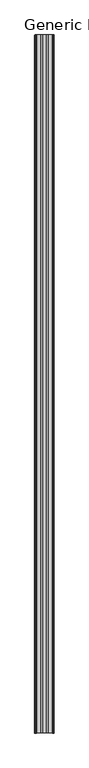
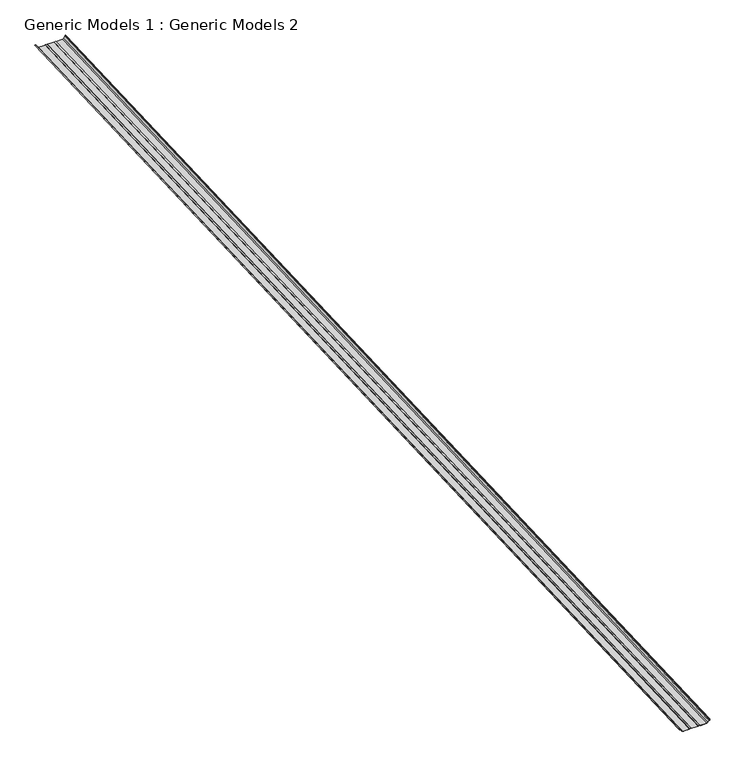
"""IFC4 building model written with IfcOpenShell, lengths in millimetres: proxy geometry, Generic Models 1 : Generic Models 2."""

import ifcopenshell
import ifcopenshell.guid

model = None  # the IFC model being written
_history = None  # IfcOwnerHistory: only IFC2X3 demands one
_inside = {}  # id of a spatial element -> (the spatial element, [elements in it])
_under = {}  # id of a project, library or spatial element -> (it, [spatial elements below it])
_declared = {}  # id of a project -> (the project, [libraries it declares])
_typed = {}  # id of a type object -> (the type object, [elements of that type])
_made_of = {}  # id of a material, layer set ... -> (it, [elements and type objects made of it])


def new_model(schema):
    """Start an empty IFC model of exactly this schema.

    Asked for "IFC4X3", IfcOpenShell would pick the latest addendum, in which some entities
    have other attributes; the version numbers below select the first issue.
    IFC2X3 requires an IfcOwnerHistory on every rooted entity: one is made here for all.
    """
    global model, _history
    if schema == "IFC4X3":
        model = ifcopenshell.file(schema_version=(4, 3, 0, 0))
    else:
        model = ifcopenshell.file(schema=schema)
    _inside.clear()
    _under.clear()
    _declared.clear()
    _typed.clear()
    _made_of.clear()
    _history = None
    if model.schema == "IFC2X3":
        org = make("IfcOrganization", Name="unknown")
        user = make(
            "IfcPersonAndOrganization",
            ThePerson=make("IfcPerson", FamilyName="unknown"),
            TheOrganization=org,
        )
        app = make(
            "IfcApplication",
            ApplicationDeveloper=org,
            Version="unknown",
            ApplicationFullName="unknown",
            ApplicationIdentifier="unknown",
        )
        _history = make(
            "IfcOwnerHistory",
            OwningUser=user,
            OwningApplication=app,
            ChangeAction="ADDED",
            CreationDate=0,
        )
    return model


def make(cls, **values):
    """One entity of the class cls with the attributes given. An attribute that is None is left unset."""
    return model.create_entity(
        cls, **{name: value for name, value in values.items() if value is not None}
    )


def rooted(cls, **values):
    """An entity with a GlobalId (a new one), such as an element, a storey or a relation."""
    return make(cls, GlobalId=ifcopenshell.guid.new(), OwnerHistory=_history, **values)


def si_unit(unit_type, name, prefix=None):
    """IfcSIUnit, for example si_unit("LENGTHUNIT", "METRE", prefix="MILLI")."""
    return make("IfcSIUnit", UnitType=unit_type, Prefix=prefix, Name=name)


def assignment(units):
    """IfcUnitAssignment: the units of a project."""
    return None if units is None else make("IfcUnitAssignment", Units=units)


def point(xyz):
    """IfcCartesianPoint."""
    return None if xyz is None else make("IfcCartesianPoint", Coordinates=xyz)


def direction(xyz):
    """IfcDirection."""
    return None if xyz is None else make("IfcDirection", DirectionRatios=xyz)


def frame(location, z_axis=None, x_axis=None):
    """IfcAxis2Placement3D, a coordinate frame: its origin and axes. An axis left out is left unset."""
    return make(
        "IfcAxis2Placement3D",
        Location=point(location),
        Axis=direction(z_axis),
        RefDirection=direction(x_axis),
    )


def origin():
    """The frame at (0, 0, 0) with its axes left unset."""
    return frame((0.0, 0.0, 0.0))


def place(relative_to, where):
    """IfcLocalPlacement: puts the frame where relative to a parent placement (None: the world)."""
    return make(
        "IfcLocalPlacement", PlacementRelTo=relative_to, RelativePlacement=where
    )


def context(
    kind, dimensions, precision=None, world=None, true_north=None, identifier=None
):
    """IfcGeometricRepresentationContext, for example the 3D "Model" context."""
    return make(
        "IfcGeometricRepresentationContext",
        ContextIdentifier=identifier,
        ContextType=kind,
        CoordinateSpaceDimension=dimensions,
        Precision=precision,
        WorldCoordinateSystem=world,
        TrueNorth=true_north,
    )


def project(units=None, contexts=None):
    """IfcProject with its units and contexts."""
    return rooted(
        "IfcProject",
        Name="project",
        RepresentationContexts=contexts,
        UnitsInContext=assignment(units),
    )


def spatial(cls, under=None, at=None, **own):
    """A site, building, storey or space (cls), placed at a placement, below another one or the project."""
    s = rooted(cls, ObjectPlacement=at, **own)
    if under is not None:
        _under.setdefault(under.id(), (under, []))[1].append(s)
    return s


def polyline(points):
    """IfcPolyline through the points."""
    return make("IfcPolyline", Points=[point(p) for p in points])


def outline(outer, holes=None, kind="AREA"):
    """IfcArbitraryClosedProfileDef: a profile drawn as a closed curve; with holes, ...WithVoids."""
    if holes is None:
        return make("IfcArbitraryClosedProfileDef", ProfileType=kind, OuterCurve=outer)
    return make(
        "IfcArbitraryProfileDefWithVoids",
        ProfileType=kind,
        OuterCurve=outer,
        InnerCurves=holes,
    )


def extrude(swept, where, along, depth):
    """IfcExtrudedAreaSolid: the profile swept, set in the frame where, extruded along a direction by depth."""
    return make(
        "IfcExtrudedAreaSolid",
        SweptArea=swept,
        Position=where,
        ExtrudedDirection=direction(along),
        Depth=depth,
    )


def shape(context_of_items, identifier, shape_type, items):
    """IfcShapeRepresentation: the items that make up one representation, for example the "Body"."""
    return make(
        "IfcShapeRepresentation",
        ContextOfItems=context_of_items,
        RepresentationIdentifier=identifier,
        RepresentationType=shape_type,
        Items=items,
    )


def source(mapping_origin, context_of_items, identifier, shape_type, items):
    """IfcRepresentationMap: a shape defined once, which mapped items show again and again."""
    return make(
        "IfcRepresentationMap",
        MappingOrigin=mapping_origin,
        MappedRepresentation=shape(context_of_items, identifier, shape_type, items),
    )


def transform(
    local_origin,
    x_axis=None,
    y_axis=None,
    z_axis=None,
    scale=None,
    scale2=None,
    scale3=None,
    uniform=True,
):
    """IfcCartesianTransformationOperator3D, or its non-uniform kind. x_axis, y_axis, z_axis: its Axis1, 2, 3."""
    if uniform:
        return make(
            "IfcCartesianTransformationOperator3D",
            Axis1=direction(x_axis),
            Axis2=direction(y_axis),
            LocalOrigin=point(local_origin),
            Scale=scale,
            Axis3=direction(z_axis),
        )
    return make(
        "IfcCartesianTransformationOperator3DnonUniform",
        Axis1=direction(x_axis),
        Axis2=direction(y_axis),
        LocalOrigin=point(local_origin),
        Scale=scale,
        Axis3=direction(z_axis),
        Scale2=scale2,
        Scale3=scale3,
    )


def mapped(mapping_source, mapping_target):
    """IfcMappedItem: shows the shape of a source again, moved by a transform."""
    return make(
        "IfcMappedItem", MappingSource=mapping_source, MappingTarget=mapping_target
    )


def made_of(thing, what):
    """Note that an element or type object is made of a material, layer set ...; save() writes the relation."""
    if what is not None:
        _made_of.setdefault(what.id(), (what, []))[1].append(thing)
    return thing


def element(
    cls,
    number,
    at=None,
    inside=None,
    cuts=None,
    type_object=None,
    material=None,
    context=None,
    identifier="Body",
    shape_type=None,
    held_by="IfcProductDefinitionShape",
    body=None,
    shapes=None,
    **own,
):
    """One element of the class cls, such as IfcWall. Its Tag is "e" and its number.

    at: its placement. inside: the storey or other place that contains it. cuts: it is an
    opening in that element (IfcRelVoidsElement). A single representation is given by context,
    identifier, shape_type and body (its items); several are given by shapes. held_by: the class
    of the entity that holds the representations. save() writes the other relations.
    """
    e = rooted(cls, Tag="e%d" % number, ObjectPlacement=at, **own)
    if body is not None:
        shapes = [shape(context, identifier, shape_type, body)]
    if shapes is not None:
        e.Representation = make(held_by, Representations=shapes)
    if inside is not None:
        _inside.setdefault(inside.id(), (inside, []))[1].append(e)
    if cuts is not None:
        rooted(
            "IfcRelVoidsElement", RelatingBuildingElement=cuts, RelatedOpeningElement=e
        )
    if type_object is not None:
        _typed.setdefault(type_object.id(), (type_object, []))[1].append(e)
    return made_of(e, material)


def aggregate(whole, parts):
    """IfcRelAggregates: a whole, such as a stair, and the parts it consists of."""
    return rooted("IfcRelAggregates", RelatingObject=whole, RelatedObjects=parts)


def save(model, path):
    """Write the relations noted so far, then the file.

    IfcRelAggregates (storeys below a building ...), IfcRelContainedInSpatialStructure (elements
    in a storey), IfcRelDefinesByType, IfcRelAssociatesMaterial and IfcRelDeclares: one each for
    every whole, place, type object, material and project.
    """
    for whole, parts in _under.values():
        aggregate(whole, parts)
    for where, things in _inside.values():
        rooted(
            "IfcRelContainedInSpatialStructure",
            RelatedElements=things,
            RelatingStructure=where,
        )
    for kind, things in _typed.values():
        rooted("IfcRelDefinesByType", RelatedObjects=things, RelatingType=kind)
    for what, things in _made_of.values():
        rooted("IfcRelAssociatesMaterial", RelatedObjects=things, RelatingMaterial=what)
    for by, libraries in _declared.values():
        rooted("IfcRelDeclares", RelatingContext=by, RelatedDefinitions=libraries)
    model.write(path)


def generic_models_1_generic_models_2_23f56264(model_context):
    return source(origin(), model_context, "Body", "SweptSolid", [
        extrude(outline(polyline([(-1.5875, 0.0), (0.0, 0.0), (0.0, -16.2527441), (24.0067186, -12.4831292), (14.9619735, 23.6899918), (43.7640409, 30.8299277), (52.0975205, 89.5519075), (79.1719273, 115.6258502), (273.2212505, 163.7300261), (278.7617463, 157.9769959), (327.4189624, 170.0389564), (329.6308632, 177.7137798), (524.274866, 225.9653748), (529.8153618, 220.2123445), (578.4725779, 232.2743051), (580.6844787, 239.9491284), (776.3953744, 288.4652026), (813.7581754, 278.4253413), (848.5981807, 230.3385881), (877.3735955, 237.4719168), (886.4950159, 201.3639399), (870.8785324, 197.4926661), (870.4965582, 199.0335268), (884.5653238, 202.5211266), (876.2215358, 235.5507742), (847.9408599, 228.5400896), (812.8027773, 277.0382539), (776.3793775, 286.8256861), (581.9560718, 238.6288011), (579.7441709, 230.9539778), (529.3077037, 218.4509468), (523.7672078, 224.2039771), (330.9024563, 176.3934525), (328.6905555, 168.7186291), (278.2540882, 156.2155982), (272.7135923, 161.9686284), (79.9667571, 114.1873348), (53.5924659, 88.7876368), (45.1853406, 29.5467121), (16.8879222, 22.5318771), (25.9678946, -13.7821306), (-1.5875, -18.1089705), (-1.5875, 0.0)])), frame((592902.4928628, -569867.8451077, 8826.9056743), z_axis=(0.0, 0.9991330730923522, 0.041630544712176844), x_axis=(0.9706209647693522, -0.010016878541720627, 0.24040508500132102)), (0.0, 0.0, 1.0), 33307.2628596),
    ])


if __name__ == "__main__":
    model = new_model("IFC4")
    model_context = context("Model", 3, world=origin())
    ifc_project = project(units=[si_unit("LENGTHUNIT", "METRE", prefix="MILLI")], contexts=[model_context])
    site = spatial("IfcSite", under=ifc_project)
    building = spatial("IfcBuilding", under=site)
    placement = place(None, origin())
    generic_models_1_generic_models_2_shape = generic_models_1_generic_models_2_23f56264(model_context)
    element("IfcBuildingElementProxy", 1, Name="Generic Models 1 : Generic Models 2", ObjectType="Generic Models 1 : Generic Models 2", at=placement, inside=building, context=model_context, shape_type="MappedRepresentation", body=[
        mapped(generic_models_1_generic_models_2_shape, transform((0.0, 0.0, 0.0), x_axis=(1.0, 0.0, 0.0), y_axis=(0.0, 1.0, 0.0), z_axis=(0.0, 0.0, 1.0))),
    ])
    save(model, "model.ifc")

# Revit data of these elements
# Element 1 (IfcBuildingElementProxy, "Generic Models 1 : Generic Models 2")
#   Materials on its faces: "STRUCTURAL STANDING SEAM SHEET METAL ROOFING - DOUBLE-LOK - COLOR T.B.D."
# Materials
#   "STRUCTURAL STANDING SEAM SHEET METAL ROOFING - DOUBLE-LOK - COLOR T.B.D.": class "Generic", colour RGB 192 192 192, transparency 0, Cost = 0
